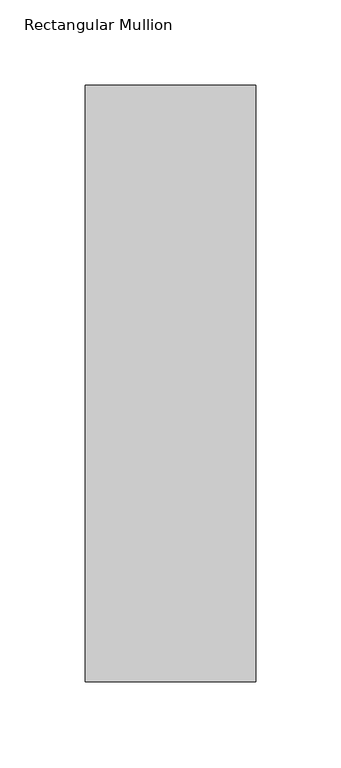
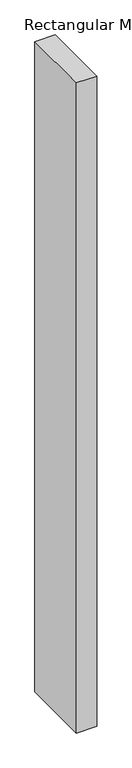
"""IFC4 building model written with IfcOpenShell, lengths in millimetres: member geometry, Rectangular Mullion : WWm-100x350-100mmOffset."""

from ifc_helpers import new_model, si_unit, frame, origin, place, context, project, spatial, polyline, outline, extrude, source, transform, mapped, element, save


def rectangular_mullion_24d91f26(model_context):
    return source(origin(), model_context, "Body", "SweptSolid", [
        extrude(outline(polyline([(50.0, 175.0), (50.0, -175.0), (-50.0, -175.0), (-50.0, 175.0), (50.0, 175.0)])), frame((0.0, 0.0, -3350.0), z_axis=(0.0, 0.0, 1.0), x_axis=(1.0, 0.0, 0.0)), (0.0, 0.0, 1.0), 3350.0),
    ])


if __name__ == "__main__":
    model = new_model("IFC4")
    model_context = context("Model", 3, world=origin())
    ifc_project = project(units=[si_unit("LENGTHUNIT", "METRE", prefix="MILLI")], contexts=[model_context])
    site = spatial("IfcSite", under=ifc_project)
    building = spatial("IfcBuilding", under=site)
    placement = place(None, origin())
    rectangular_mullion_shape = rectangular_mullion_24d91f26(model_context)
    element("IfcMember", 1, ObjectType="Rectangular Mullion : WWm-100x350-100mmOffset", at=placement, inside=building, context=model_context, shape_type="MappedRepresentation", body=[
        mapped(rectangular_mullion_shape, transform((0.0, 0.0, 0.0), x_axis=(1.0, 0.0, 0.0), y_axis=(0.0, 1.0, 0.0), z_axis=(0.0, 0.0, 1.0))),
    ])
    save(model, "model.ifc")

# Revit data of these elements
# Type "Rectangular Mullion : WWm-100x350-100mmOffset"
#   built-in parameter 1007304 = 1.14829 (stored number, unit not read)
#   built-in parameter 1007301 = 0.164042 (stored number, unit not read)
#   built-in parameter 1007300 = 0.164042 (stored number, unit not read)
# Element 1 (IfcMember, "Rectangular Mullion : WWm-100x350-100mmOffset")
#   Materials on its faces: "WW-EC-RGB-Mullion"
# Materials
#   "WW-EC-RGB-Mullion": class "Generic", colour RGB 255 255 255, transparency 0, Comments = "If region requests black mullions, switch asset color to RGB 25-25-25", Description = "Generic Color", Cost = 0
